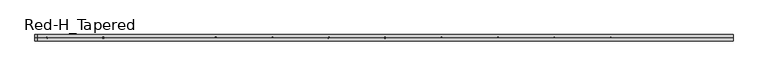
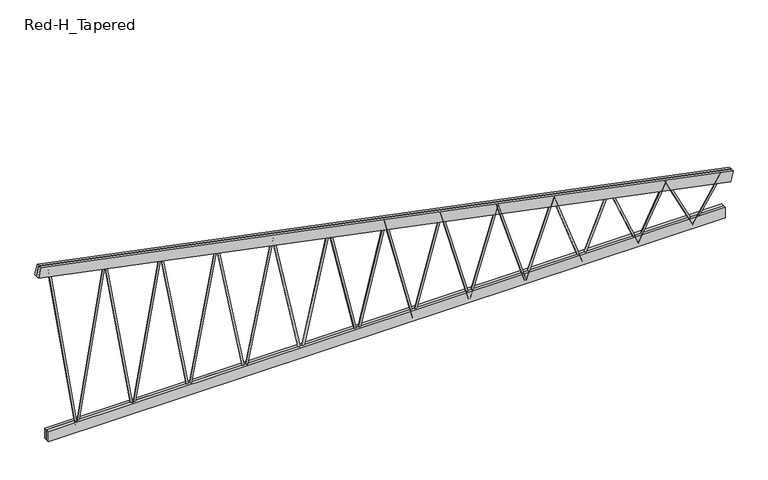
"""IFC4 building model written with IfcOpenShell, lengths in millimetres: beam geometry, Construction_Frames_RedBuilt_Openweb_Red-H_Tapered : Red-H_Tapered."""

from ifc_helpers import new_model, si_unit, point, frame, origin, origin_2d, place, context, project, spatial, polyline, circle_curve, trimmed, segment, composite_curve, outline, extrude, source, transform, mapped, element, save


def red_h_tapered_00fe0e34(model_context):
    return source(origin(), model_context, "Body", "SweptSolid", [
        extrude(outline(composite_curve([segment(trimmed(circle_curve(origin_2d(), 12.7), [point((0.0, 12.6999999))], [point((0.0, -12.7))], False, "CARTESIAN"), True, "CONTINUOUS"), segment(trimmed(circle_curve(origin_2d(), 12.7), [point((0.0, -12.7))], [point((0.0, 12.6999999))], False, "CARTESIAN"), True, "CONTINUOUS")], self_intersect=False)), frame((-4030.9270833, 0.0, -367.0101562), z_axis=(-0.15460396667959522, 0.0, 0.9879765247651052), x_axis=(0.0, -1.0, 0.0)), (0.0, 0.0, 1.0), 2370.2361882),
        extrude(outline(composite_curve([segment(trimmed(circle_curve(origin_2d(), 12.7), [point((0.0, -12.7))], [point((0.0, 12.7))], False, "CARTESIAN"), True, "CONTINUOUS"), segment(trimmed(circle_curve(origin_2d(), 12.7), [point((0.0, 12.7))], [point((0.0, -12.7))], False, "CARTESIAN"), True, "CONTINUOUS")], self_intersect=False)), frame((1099.34375, 0.0, -367.0101562), z_axis=(-0.2681543031579758, 0.0, 0.9633759752546565), x_axis=(0.0, -1.0, 0.0)), (0.0, 0.0, 1.0), 1366.5561669),
        extrude(outline(composite_curve([segment(trimmed(circle_curve(origin_2d(), 12.7), [point((0.0, 12.7))], [point((0.0, -12.7))], False, "CARTESIAN"), True, "CONTINUOUS"), segment(trimmed(circle_curve(origin_2d(), 12.7), [point((0.0, -12.7))], [point((0.0, 12.7))], False, "CARTESIAN"), True, "CONTINUOUS")], self_intersect=False)), frame((366.4479167, 0.0, -367.0101562), z_axis=(0.2681543031579784, 0.0, 0.9633759752546557), x_axis=(0.0, -1.0, 0.0)), (0.0, 0.0, 1.0), 1366.5561669),
        extrude(outline(composite_curve([segment(trimmed(circle_curve(origin_2d(), 12.7), [point((0.0, -12.7000001))], [point((0.0, 12.7))], False, "CARTESIAN"), True, "CONTINUOUS"), segment(trimmed(circle_curve(origin_2d(), 12.7), [point((0.0, 12.7))], [point((0.0, -12.7000001))], False, "CARTESIAN"), True, "CONTINUOUS")], self_intersect=False)), frame((366.4479167, 0.0, -367.0101562), z_axis=(-0.24297599661504005, 0.0, 0.9700323010441085), x_axis=(0.0, -1.0, 0.0)), (0.0, 0.0, 1.0), 1508.1650936),
        extrude(outline(composite_curve([segment(trimmed(circle_curve(origin_2d(), 12.7), [point((0.0, 12.7000001))], [point((0.0, -12.7))], False, "CARTESIAN"), True, "CONTINUOUS"), segment(trimmed(circle_curve(origin_2d(), 12.7), [point((0.0, -12.7))], [point((0.0, 12.7000001))], False, "CARTESIAN"), True, "CONTINUOUS")], self_intersect=False)), frame((-366.4479167, 0.0, -367.0101562), z_axis=(0.24297599661500857, 0.0, 0.9700323010441164), x_axis=(0.0, -1.0, 0.0)), (0.0, 0.0, 1.0), 1508.1650936),
        extrude(outline(composite_curve([segment(trimmed(circle_curve(origin_2d(), 12.7), [point((0.0, -12.7))], [point((0.0, 12.7))], False, "CARTESIAN"), True, "CONTINUOUS"), segment(trimmed(circle_curve(origin_2d(), 12.7), [point((0.0, 12.7))], [point((0.0, -12.7))], False, "CARTESIAN"), True, "CONTINUOUS")], self_intersect=False)), frame((-366.4479167, 0.0, -367.0101562), z_axis=(-0.2220060758096705, 0.0, 0.9750452821810847), x_axis=(0.0, -1.0, 0.0)), (0.0, 0.0, 1.0), 1650.6211162),
        extrude(outline(composite_curve([segment(trimmed(circle_curve(origin_2d(), 12.7), [point((0.0, 12.7))], [point((0.0, -12.7))], False, "CARTESIAN"), True, "CONTINUOUS"), segment(trimmed(circle_curve(origin_2d(), 12.7), [point((0.0, -12.7))], [point((0.0, 12.7))], False, "CARTESIAN"), True, "CONTINUOUS")], self_intersect=False)), frame((-1099.34375, 0.0, -367.0101562), z_axis=(0.22200607580967185, 0.0, 0.9750452821810842), x_axis=(0.0, -1.0, 0.0)), (0.0, 0.0, 1.0), 1650.6211162),
        extrude(outline(composite_curve([segment(trimmed(circle_curve(origin_2d(), 12.7), [point((0.0, -12.7))], [point((0.0, 12.7))], False, "CARTESIAN"), True, "CONTINUOUS"), segment(trimmed(circle_curve(origin_2d(), 12.7), [point((0.0, 12.7))], [point((0.0, -12.7))], False, "CARTESIAN"), True, "CONTINUOUS")], self_intersect=False)), frame((-1099.34375, 0.0, -367.0101562), z_axis=(-0.20429466272790736, 0.0, 0.97890943951976), x_axis=(0.0, -1.0, 0.0)), (0.0, 0.0, 1.0), 1793.7224192),
        extrude(outline(composite_curve([segment(trimmed(circle_curve(origin_2d(), 12.7), [point((0.0, -12.7))], [point((0.0, 12.6999999))], False, "CARTESIAN"), True, "CONTINUOUS"), segment(trimmed(circle_curve(origin_2d(), 12.7), [point((0.0, 12.6999999))], [point((0.0, -12.7))], False, "CARTESIAN"), True, "CONTINUOUS")], self_intersect=False)), frame((-1832.2395833, 0.0, -367.0101562), z_axis=(0.2042946627279104, 0.0, 0.9789094395197594), x_axis=(0.0, -1.0, 0.0)), (0.0, 0.0, 1.0), 1793.7224192),
        extrude(outline(composite_curve([segment(trimmed(circle_curve(origin_2d(), 12.7), [point((0.0, 12.7))], [point((0.0, -12.7))], False, "CARTESIAN"), True, "CONTINUOUS"), segment(trimmed(circle_curve(origin_2d(), 12.7), [point((0.0, -12.7))], [point((0.0, 12.7))], False, "CARTESIAN"), True, "CONTINUOUS")], self_intersect=False)), frame((-1832.2395833, 0.0, -367.0101562), z_axis=(-0.1891513940348578, 0.0, 0.9819479365703001), x_axis=(0.0, -1.0, 0.0)), (0.0, 0.0, 1.0), 1937.3260162),
        extrude(outline(composite_curve([segment(trimmed(circle_curve(origin_2d(), 12.7), [point((0.0, -12.7))], [point((0.0, 12.7))], False, "CARTESIAN"), True, "CONTINUOUS"), segment(trimmed(circle_curve(origin_2d(), 12.7), [point((0.0, 12.7))], [point((0.0, -12.7))], False, "CARTESIAN"), True, "CONTINUOUS")], self_intersect=False)), frame((-2565.1354167, 0.0, -367.0101562), z_axis=(0.18915139403485653, 0.0, 0.9819479365703003), x_axis=(0.0, -1.0, 0.0)), (0.0, 0.0, 1.0), 1937.3260162),
        extrude(outline(composite_curve([segment(trimmed(circle_curve(origin_2d(), 12.7), [point((0.0, 12.7))], [point((0.0, -12.6999999))], False, "CARTESIAN"), True, "CONTINUOUS"), segment(trimmed(circle_curve(origin_2d(), 12.7), [point((0.0, -12.6999999))], [point((0.0, 12.7))], False, "CARTESIAN"), True, "CONTINUOUS")], self_intersect=False)), frame((-2565.1354167, 0.0, -367.0101562), z_axis=(-0.17606447763370592, 0.0, 0.9843786363567478), x_axis=(0.0, -1.0, 0.0)), (0.0, 0.0, 1.0), 2081.3279407),
        extrude(outline(composite_curve([segment(trimmed(circle_curve(origin_2d(), 12.7), [point((0.0, -12.7))], [point((0.0, 12.7))], False, "CARTESIAN"), True, "CONTINUOUS"), segment(trimmed(circle_curve(origin_2d(), 12.7), [point((0.0, 12.7))], [point((0.0, -12.7))], False, "CARTESIAN"), True, "CONTINUOUS")], self_intersect=False)), frame((-3298.03125, 0.0, -367.0101562), z_axis=(0.17606447763370967, 0.0, 0.9843786363567472), x_axis=(0.0, -1.0, 0.0)), (0.0, 0.0, 1.0), 2081.3279407),
        extrude(outline(composite_curve([segment(trimmed(circle_curve(origin_2d(), 12.7), [point((0.0, 12.7))], [point((0.0, -12.7))], False, "CARTESIAN"), True, "CONTINUOUS"), segment(trimmed(circle_curve(origin_2d(), 12.7), [point((0.0, -12.7))], [point((0.0, 12.7))], False, "CARTESIAN"), True, "CONTINUOUS")], self_intersect=False)), frame((-3298.03125, 0.0, -367.0101562), z_axis=(-0.16464752867330681, 0.0, 0.9863524680872313), x_axis=(0.0, -1.0, 0.0)), (0.0, 0.0, 1.0), 2225.6508775),
        extrude(outline(composite_curve([segment(trimmed(circle_curve(origin_2d(), 12.7), [point((0.0, -12.7000001))], [point((0.0, 12.7))], False, "CARTESIAN"), True, "CONTINUOUS"), segment(trimmed(circle_curve(origin_2d(), 12.7), [point((0.0, 12.7))], [point((0.0, -12.7000001))], False, "CARTESIAN"), True, "CONTINUOUS")], self_intersect=False)), frame((-4030.9270833, 0.0, -367.0101562), z_axis=(0.16464752867330554, 0.0, 0.9863524680872315), x_axis=(0.0, -1.0, 0.0)), (0.0, 0.0, 1.0), 2225.6508775),
        extrude(outline(composite_curve([segment(trimmed(circle_curve(origin_2d(), 12.7), [point((0.0, 12.7000001))], [point((0.0, -12.6999999))], False, "CARTESIAN"), True, "CONTINUOUS"), segment(trimmed(circle_curve(origin_2d(), 12.7), [point((0.0, -12.6999999))], [point((0.0, 12.7000001))], False, "CARTESIAN"), True, "CONTINUOUS")], self_intersect=False)), frame((4030.9270833, 0.0, -367.0101562), z_axis=(0.5313777127822298, 0.0, 0.8471350107027369), x_axis=(0.0, -1.0, 0.0)), (0.0, 0.0, 1.0), 689.6185291),
        extrude(outline(composite_curve([segment(trimmed(circle_curve(origin_2d(), 12.7), [point((0.0, -12.7))], [point((0.0, 12.7))], False, "CARTESIAN"), True, "CONTINUOUS"), segment(trimmed(circle_curve(origin_2d(), 12.7), [point((0.0, 12.7))], [point((0.0, -12.7))], False, "CARTESIAN"), True, "CONTINUOUS")], self_intersect=False)), frame((4030.9270833, 0.0, -367.0101562), z_axis=(-0.4483066524741803, 0.0, 0.8938798271285658), x_axis=(0.0, -1.0, 0.0)), (0.0, 0.0, 1.0), 817.4045927),
        extrude(outline(composite_curve([segment(trimmed(circle_curve(origin_2d(), 12.7), [point((0.0, 12.7))], [point((0.0, -12.7))], False, "CARTESIAN"), True, "CONTINUOUS"), segment(trimmed(circle_curve(origin_2d(), 12.7), [point((0.0, -12.7))], [point((0.0, 12.7))], False, "CARTESIAN"), True, "CONTINUOUS")], self_intersect=False)), frame((3298.03125, 0.0, -367.0101562), z_axis=(0.44830665247417884, 0.0, 0.8938798271285665), x_axis=(0.0, -1.0, 0.0)), (0.0, 0.0, 1.0), 817.4045927),
        extrude(outline(composite_curve([segment(trimmed(circle_curve(origin_2d(), 12.7), [point((0.0, -12.7000001))], [point((0.0, 12.7))], False, "CARTESIAN"), True, "CONTINUOUS"), segment(trimmed(circle_curve(origin_2d(), 12.7), [point((0.0, 12.7))], [point((0.0, -12.7000001))], False, "CARTESIAN"), True, "CONTINUOUS")], self_intersect=False)), frame((3298.03125, 0.0, -367.0101562), z_axis=(-0.3854936577351087, 0.0, 0.9227104853885681), x_axis=(0.0, -1.0, 0.0)), (0.0, 0.0, 1.0), 950.5938926),
        extrude(outline(composite_curve([segment(trimmed(circle_curve(origin_2d(), 12.7), [point((0.0, 12.7))], [point((0.0, -12.7))], False, "CARTESIAN"), True, "CONTINUOUS"), segment(trimmed(circle_curve(origin_2d(), 12.7), [point((0.0, -12.7))], [point((0.0, 12.7))], False, "CARTESIAN"), True, "CONTINUOUS")], self_intersect=False)), frame((2565.1354167, 0.0, -367.0101562), z_axis=(0.38549365773510985, 0.0, 0.9227104853885676), x_axis=(0.0, -1.0, 0.0)), (0.0, 0.0, 1.0), 950.5938926),
        extrude(outline(composite_curve([segment(trimmed(circle_curve(origin_2d(), 12.7), [point((0.0, -12.7000001))], [point((0.0, 12.7))], False, "CARTESIAN"), True, "CONTINUOUS"), segment(trimmed(circle_curve(origin_2d(), 12.7), [point((0.0, 12.7))], [point((0.0, -12.7000001))], False, "CARTESIAN"), True, "CONTINUOUS")], self_intersect=False)), frame((2565.1354167, 0.0, -367.0101562), z_axis=(-0.33705582458152517, 0.0, 0.9414846632397514), x_axis=(0.0, -1.0, 0.0)), (0.0, 0.0, 1.0), 1087.2024452),
        extrude(outline(composite_curve([segment(trimmed(circle_curve(origin_2d(), 12.7), [point((0.0, 12.7000001))], [point((0.0, -12.7))], False, "CARTESIAN"), True, "CONTINUOUS"), segment(trimmed(circle_curve(origin_2d(), 12.7), [point((0.0, -12.7))], [point((0.0, 12.7000001))], False, "CARTESIAN"), True, "CONTINUOUS")], self_intersect=False)), frame((1832.2395833, 0.0, -367.0101562), z_axis=(0.33705582458152494, 0.0, 0.9414846632397516), x_axis=(0.0, -1.0, 0.0)), (0.0, 0.0, 1.0), 1087.2024452),
        extrude(outline(composite_curve([segment(trimmed(circle_curve(origin_2d(), 12.7), [point((0.0, -12.7))], [point((0.0, 12.7))], False, "CARTESIAN"), True, "CONTINUOUS"), segment(trimmed(circle_curve(origin_2d(), 12.7), [point((0.0, 12.7))], [point((0.0, -12.7))], False, "CARTESIAN"), True, "CONTINUOUS")], self_intersect=False)), frame((1832.2395833, 0.0, -367.0101562), z_axis=(-0.29887573492329583, 0.0, 0.9542920386726801), x_axis=(0.0, -1.0, 0.0)), (0.0, 0.0, 1.0), 1226.0878815),
        extrude(outline(composite_curve([segment(trimmed(circle_curve(origin_2d(), 12.7), [point((0.0, 12.7))], [point((0.0, -12.7))], False, "CARTESIAN"), True, "CONTINUOUS"), segment(trimmed(circle_curve(origin_2d(), 12.7), [point((0.0, -12.7))], [point((0.0, 12.7))], False, "CARTESIAN"), True, "CONTINUOUS")], self_intersect=False)), frame((1099.34375, 0.0, -367.0101562), z_axis=(0.29887573492329916, 0.0, 0.954292038672679), x_axis=(0.0, -1.0, 0.0)), (0.0, 0.0, 1.0), 1226.0878815),
        extrude(outline(polyline([(-4422.775, -41.275), (-4422.775, -3.175), (4422.775, -3.175), (4422.775, -41.275), (-4422.775, -41.275)])), frame((0.0, 0.0, -386.0601562), z_axis=(0.0, 0.0, 1.0), x_axis=(1.0, 0.0, 0.0)), (0.0, 0.0, 1.0), 139.7),
        extrude(outline(polyline([(-4422.775, 3.175), (-4422.775, 41.275), (4422.775, 41.275), (4422.775, 3.175), (-4422.775, 3.175)])), frame((0.0, 0.0, -386.0601562), z_axis=(0.0, 0.0, 1.0), x_axis=(1.0, 0.0, 0.0)), (0.0, 0.0, 1.0), 139.7),
        extrude(outline(polyline([(0.0, -38.1), (0.0, 0.0), (9231.7054764, 0.0), (9231.7054764, -38.1), (0.0, -38.1)])), frame((-4552.0495571, -3.175, 1915.4084416), z_axis=(0.19809990739852568, 0.0, 0.9801818334822858), x_axis=(0.9801818334822858, 0.0, -0.19809990739852568)), (0.0, 0.0, 1.0), 139.7),
        extrude(outline(polyline([(0.0, -38.1), (0.0, 0.0), (9231.7054764, 0.0), (9231.7054764, -38.1), (0.0, -38.1)])), frame((-4552.0495571, 41.275, 1915.4084416), z_axis=(0.19809990739852568, 0.0, 0.9801818334822858), x_axis=(0.9801818334822858, 0.0, -0.19809990739852568)), (0.0, 0.0, 1.0), 139.7),
    ])


if __name__ == "__main__":
    model = new_model("IFC4")
    model_context = context("Model", 3, world=origin())
    ifc_project = project(units=[si_unit("LENGTHUNIT", "METRE", prefix="MILLI")], contexts=[model_context])
    site = spatial("IfcSite", under=ifc_project)
    building = spatial("IfcBuilding", under=site)
    placement = place(None, origin())
    red_h_tapered_shape = red_h_tapered_00fe0e34(model_context)
    element("IfcBeam", 1, ObjectType="Construction_Frames_RedBuilt_Openweb_Red-H_Tapered : Red-H_Tapered", at=placement, inside=building, context=model_context, shape_type="MappedRepresentation", body=[
        mapped(red_h_tapered_shape, transform((0.0, 0.0, 0.0), x_axis=(1.0, 0.0, 0.0), y_axis=(0.0, 1.0, 0.0), z_axis=(0.0, 0.0, 1.0))),
    ])
    save(model, "model.ifc")

# Revit data of these elements
# Project information
#   Project Issue Date = "02/27/2019"
#   Project Status = "Project Status"
#   Client Name = "Owner"
#   Project Address = "714 N WATERTOWN AVE., JEFFERSON, WI"
#   Project Name = "LEGACY AUTO SALES"
#   Project Number = "Project Number"
# Type "Construction_Frames_RedBuilt_Openweb_Red-H_Tapered : Red-H_Tapered"
#   Youtube clip = ""
#   Weight Net (Kg) = "0"
#   Webs = "Up to 2\" diameter tubular steel"
#   Uniformat II Description = ""
#   Uniformat II Code = ""
#   Uniclass 2015 Name = "Softwood trusses"
#   Uniclass 2015 Code = "Pr_20_85_90_81"
#   Uniclass 2.0 Description = "Structural Framing Systems"
#   Uniclass 2.0 Code = "SS-15-10-75"
#   Uniclass 1.4 Description = "Trusses"
#   Uniclass 1.4 Code = "L3523"
#   UNSPSC Code = "30103606"
#   Technical description = "http://www.redbuilt.com/reference/literature-and-other-resources"
#   Region South America = "None"
#   Region Oceania = "None"
#   Region North America = "US"
#   Region Middle East = "None"
#   Region Europe = "None"
#   Region Asia = "None"
#   Region Antarctica = "None"
#   Region Africa = "None"
#   QR code = "http://bimobject.com/redbuilt/product/redbuilt-0003"
#   Product url = "http://www.redbuilt.com/products/default.aspx?id=2"
#   Product group = "Wood Trusses"
#   Product family = "Construction"
#   Product data url = "https://bimobject.com/redbuilt/product/redbuilt-0003"
#   Product certification = ""
#   Product SKU = "redbuilt-0003"
#   Product Page URL = "http://www.redbuilt.com/commercial-systems/red-m-red-h-open-web-trusses"
#   Product Guid = "2c5793f2-6ffb-4665-b825-cf90c048e711"
#   Product Documentation Link = "http://www.redbuilt.com/documents/OW_Guide_2017_07_LowRes_wLinks.pdf"
#   OmniClass Description = "Wood Trusses"
#   OmniClass Code = "23-13 35 19 13 17"
#   NBS Reference Description = ""
#   NBS Reference Code = ""
#   Material secondary = "Steel"
#   Material main = "Wood"
#   Masterformat 2014 Description = "Metal-Web Wood Joists"
#   Masterformat 2014 Code = "06 17 36"
#   Manufacturer name = "RedBuilt"
#   Manufacturer country = "United States"
#   Installation instructions = "http://www.redbuilt.com/documents/Installation_Sheets_Open-Web.pdf"
#   IFC Classification = ""
#   EAN code = ""
#   Design country = "United States"
#   Product Information = "http://redbuilt.com/products/default.aspx?id=2"
#   Model = "Red-H-Tapered"
#   Manufacturer URL = "http://redbuilt.com/"
#   Manufacturer = "RedBuilt™"
#   Description = "Open Web Truss"
#   Date of publishing = "8/17/2010"
#   Contact us = "http://redbuilt.com/contact/"
#   Chords = "Double 1½\" x 5½\" MSR lumber"
#   COBIe Type Category = ""
#   Brand url = "http://www.redbuilt.com"
#   BIMobject main category code = "construction"
#   BIMobject main category = "Construction"
#   BIMobject category code = "construction-frames-trusses"
#   BIMobject category = "Frames & Trusses"
#   Web Radius = 0' - 0 1/2"
#   Web Layout Offset Start [instance default] = 0' - 5"
#   Web Layout Offset End [instance default] = 0' - 5"
#   Web Diameter = 0' - 1"
#   TotalLength [instance default] = 20' - 0"
#   Span Minimum = 4' - 0"
#   Span Maximum = 70' - 0"
#   Span Limit [instance default] = 20' - 0"
#   Nominal width = 0' - 0"
#   Nominal height = 0' - 0"
#   Inner Depth Top [instance default] = 0' - 2.76372"
#   Depth Start [instance default] = 6' - 0"
#   Top Chord Length [instance default] = 20' - 1.19701"
#   TC Extension Start Aux [instance default] = 0' - 0"
#   TC Extension End Aux [instance default] = 0' - 0"
#   T-B Chord Length Difference L [instance default] = 0' - 4"
#   T-B Chord Length Difference [instance default] = 0' - 4"
#   Height 2 [instance default] = 6' - 0"
#   Depth Minimum at Wall = 2' - 0"
#   Depth Maximum at Wall = 6' - 0"
#   Depth Lower End [instance default] = 2' - 0"
#   Depth Higher End [instance default] = 6' - 0"
#   Depth End [instance default] = 2' - 0"
#   Depth 2 [instance default] = 2' - 0"
#   Chord Width = 0' - 3 1/4"
#   Chord Thickness = 0' - 1 1/2"
#   Chord Depth = 0' - 5 1/2"
#   Offset Start [instance default] = 0' - 0"
#   TC Extension Start [instance default] = 0' - 0"
#   End Panel = 0' - 5"
#   Offset End [instance default] = 0' - 0"
#   TC Extension End [instance default] = 0' - 0"
#   Length [instance default] = 20' - 0"
#   Angle [instance default] = 5.71059°
#   Span Limit Warning [instance default] = no
#   Edition number = 1
#   Top Bearing Start [instance default] = yes
#   Top Bearing End [instance default] = yes
#   Bottom Bearing Start [instance default] = no
#   Bottom Bearing End [instance default] = no
#   8 Panels [instance default] = yes
#   16 Panels [instance default] = no
#   12 Panels [instance default] = no
#   Web Material = RedBuilt-Steel, Galvanized
#   Clip Material = RedBuilt-Steel, Galvanized
#   Chords Material = RedBuilt-MSR
#   URL = ""
#   Assembly Code = ""
# Element 1 (IfcBeam, "Construction_Frames_RedBuilt_Openweb_Red-H_Tapered : Red-H_Tapered")
#   TotalLength = 29' - 8 1/4"
#   Span Limit = 29' - 8 1/4"
#   Inner Depth Top = 0' - 2.8056"
#   Top Chord Length = 30' - 3.45297"
#   Depth 2 = 6' - 0"
#   Angle = 11.4259°
#   8 Panels = no
#   12 Panels = yes
#   Materials on its faces: "RedBuilt-Steel, Galvanized", "RedBuilt-MSR"
# Materials
#   "RedBuilt-Steel, Galvanized": class "Metal", colour RGB 164 172 176, transparency 0, Manufacturer = "RedBuilt. LLC", Comments = "Openweb Metal Web", URL = "http://www.redbuilt.com/", Description = "Galvanized steel", Cost = 0
#   "RedBuilt-MSR": class "Wood", colour RGB 213 182 136, transparency 0, Manufacturer = "RedBuilt, LLC", URL = "http://www.redbuilt.com/", Cost = 0
